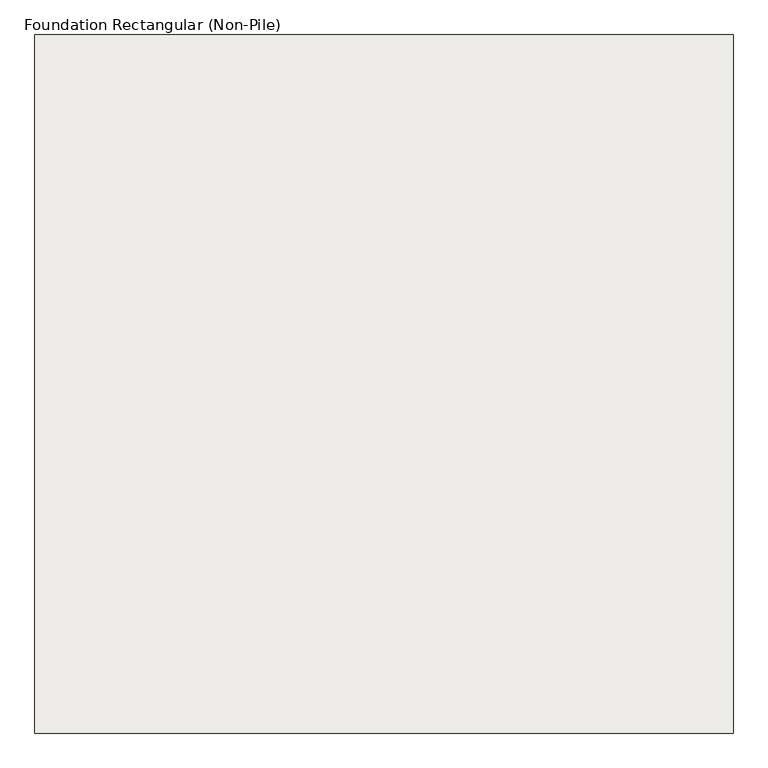
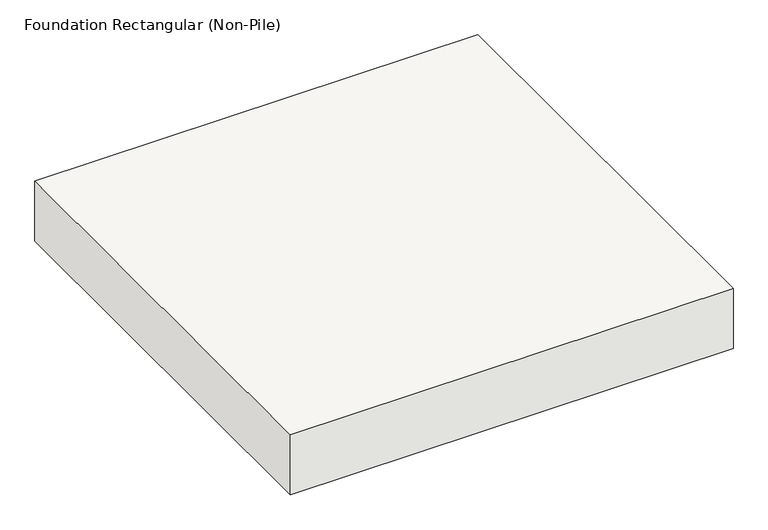
"""IFC4 building model written with IfcOpenShell, lengths in millimetres: slab geometry, Foundation Rectangular (Non-Pile) : H_SF_AR S18_Ret Fdn_F3 3500x3500x600."""

import ifcopenshell
import ifcopenshell.guid

model = None  # the IFC model being written
_history = None  # IfcOwnerHistory: only IFC2X3 demands one
_inside = {}  # id of a spatial element -> (the spatial element, [elements in it])
_under = {}  # id of a project, library or spatial element -> (it, [spatial elements below it])
_declared = {}  # id of a project -> (the project, [libraries it declares])
_typed = {}  # id of a type object -> (the type object, [elements of that type])
_made_of = {}  # id of a material, layer set ... -> (it, [elements and type objects made of it])


def new_model(schema):
    """Start an empty IFC model of exactly this schema.

    Asked for "IFC4X3", IfcOpenShell would pick the latest addendum, in which some entities
    have other attributes; the version numbers below select the first issue.
    IFC2X3 requires an IfcOwnerHistory on every rooted entity: one is made here for all.
    """
    global model, _history
    if schema == "IFC4X3":
        model = ifcopenshell.file(schema_version=(4, 3, 0, 0))
    else:
        model = ifcopenshell.file(schema=schema)
    _inside.clear()
    _under.clear()
    _declared.clear()
    _typed.clear()
    _made_of.clear()
    _history = None
    if model.schema == "IFC2X3":
        org = make("IfcOrganization", Name="unknown")
        user = make(
            "IfcPersonAndOrganization",
            ThePerson=make("IfcPerson", FamilyName="unknown"),
            TheOrganization=org,
        )
        app = make(
            "IfcApplication",
            ApplicationDeveloper=org,
            Version="unknown",
            ApplicationFullName="unknown",
            ApplicationIdentifier="unknown",
        )
        _history = make(
            "IfcOwnerHistory",
            OwningUser=user,
            OwningApplication=app,
            ChangeAction="ADDED",
            CreationDate=0,
        )
    return model


def make(cls, **values):
    """One entity of the class cls with the attributes given. An attribute that is None is left unset."""
    return model.create_entity(
        cls, **{name: value for name, value in values.items() if value is not None}
    )


def rooted(cls, **values):
    """An entity with a GlobalId (a new one), such as an element, a storey or a relation."""
    return make(cls, GlobalId=ifcopenshell.guid.new(), OwnerHistory=_history, **values)


def si_unit(unit_type, name, prefix=None):
    """IfcSIUnit, for example si_unit("LENGTHUNIT", "METRE", prefix="MILLI")."""
    return make("IfcSIUnit", UnitType=unit_type, Prefix=prefix, Name=name)


def assignment(units):
    """IfcUnitAssignment: the units of a project."""
    return None if units is None else make("IfcUnitAssignment", Units=units)


def point(xyz):
    """IfcCartesianPoint."""
    return None if xyz is None else make("IfcCartesianPoint", Coordinates=xyz)


def direction(xyz):
    """IfcDirection."""
    return None if xyz is None else make("IfcDirection", DirectionRatios=xyz)


def frame(location, z_axis=None, x_axis=None):
    """IfcAxis2Placement3D, a coordinate frame: its origin and axes. An axis left out is left unset."""
    return make(
        "IfcAxis2Placement3D",
        Location=point(location),
        Axis=direction(z_axis),
        RefDirection=direction(x_axis),
    )


def origin():
    """The frame at (0, 0, 0) with its axes left unset."""
    return frame((0.0, 0.0, 0.0))


def place(relative_to, where):
    """IfcLocalPlacement: puts the frame where relative to a parent placement (None: the world)."""
    return make(
        "IfcLocalPlacement", PlacementRelTo=relative_to, RelativePlacement=where
    )


def context(
    kind, dimensions, precision=None, world=None, true_north=None, identifier=None
):
    """IfcGeometricRepresentationContext, for example the 3D "Model" context."""
    return make(
        "IfcGeometricRepresentationContext",
        ContextIdentifier=identifier,
        ContextType=kind,
        CoordinateSpaceDimension=dimensions,
        Precision=precision,
        WorldCoordinateSystem=world,
        TrueNorth=true_north,
    )


def project(units=None, contexts=None):
    """IfcProject with its units and contexts."""
    return rooted(
        "IfcProject",
        Name="project",
        RepresentationContexts=contexts,
        UnitsInContext=assignment(units),
    )


def spatial(cls, under=None, at=None, **own):
    """A site, building, storey or space (cls), placed at a placement, below another one or the project."""
    s = rooted(cls, ObjectPlacement=at, **own)
    if under is not None:
        _under.setdefault(under.id(), (under, []))[1].append(s)
    return s


def polyline(points):
    """IfcPolyline through the points."""
    return make("IfcPolyline", Points=[point(p) for p in points])


def outline(outer, holes=None, kind="AREA"):
    """IfcArbitraryClosedProfileDef: a profile drawn as a closed curve; with holes, ...WithVoids."""
    if holes is None:
        return make("IfcArbitraryClosedProfileDef", ProfileType=kind, OuterCurve=outer)
    return make(
        "IfcArbitraryProfileDefWithVoids",
        ProfileType=kind,
        OuterCurve=outer,
        InnerCurves=holes,
    )


def extrude(swept, where, along, depth):
    """IfcExtrudedAreaSolid: the profile swept, set in the frame where, extruded along a direction by depth."""
    return make(
        "IfcExtrudedAreaSolid",
        SweptArea=swept,
        Position=where,
        ExtrudedDirection=direction(along),
        Depth=depth,
    )


def shape(context_of_items, identifier, shape_type, items):
    """IfcShapeRepresentation: the items that make up one representation, for example the "Body"."""
    return make(
        "IfcShapeRepresentation",
        ContextOfItems=context_of_items,
        RepresentationIdentifier=identifier,
        RepresentationType=shape_type,
        Items=items,
    )


def source(mapping_origin, context_of_items, identifier, shape_type, items):
    """IfcRepresentationMap: a shape defined once, which mapped items show again and again."""
    return make(
        "IfcRepresentationMap",
        MappingOrigin=mapping_origin,
        MappedRepresentation=shape(context_of_items, identifier, shape_type, items),
    )


def transform(
    local_origin,
    x_axis=None,
    y_axis=None,
    z_axis=None,
    scale=None,
    scale2=None,
    scale3=None,
    uniform=True,
):
    """IfcCartesianTransformationOperator3D, or its non-uniform kind. x_axis, y_axis, z_axis: its Axis1, 2, 3."""
    if uniform:
        return make(
            "IfcCartesianTransformationOperator3D",
            Axis1=direction(x_axis),
            Axis2=direction(y_axis),
            LocalOrigin=point(local_origin),
            Scale=scale,
            Axis3=direction(z_axis),
        )
    return make(
        "IfcCartesianTransformationOperator3DnonUniform",
        Axis1=direction(x_axis),
        Axis2=direction(y_axis),
        LocalOrigin=point(local_origin),
        Scale=scale,
        Axis3=direction(z_axis),
        Scale2=scale2,
        Scale3=scale3,
    )


def mapped(mapping_source, mapping_target):
    """IfcMappedItem: shows the shape of a source again, moved by a transform."""
    return make(
        "IfcMappedItem", MappingSource=mapping_source, MappingTarget=mapping_target
    )


def made_of(thing, what):
    """Note that an element or type object is made of a material, layer set ...; save() writes the relation."""
    if what is not None:
        _made_of.setdefault(what.id(), (what, []))[1].append(thing)
    return thing


def element(
    cls,
    number,
    at=None,
    inside=None,
    cuts=None,
    type_object=None,
    material=None,
    context=None,
    identifier="Body",
    shape_type=None,
    held_by="IfcProductDefinitionShape",
    body=None,
    shapes=None,
    **own,
):
    """One element of the class cls, such as IfcWall. Its Tag is "e" and its number.

    at: its placement. inside: the storey or other place that contains it. cuts: it is an
    opening in that element (IfcRelVoidsElement). A single representation is given by context,
    identifier, shape_type and body (its items); several are given by shapes. held_by: the class
    of the entity that holds the representations. save() writes the other relations.
    """
    e = rooted(cls, Tag="e%d" % number, ObjectPlacement=at, **own)
    if body is not None:
        shapes = [shape(context, identifier, shape_type, body)]
    if shapes is not None:
        e.Representation = make(held_by, Representations=shapes)
    if inside is not None:
        _inside.setdefault(inside.id(), (inside, []))[1].append(e)
    if cuts is not None:
        rooted(
            "IfcRelVoidsElement", RelatingBuildingElement=cuts, RelatedOpeningElement=e
        )
    if type_object is not None:
        _typed.setdefault(type_object.id(), (type_object, []))[1].append(e)
    return made_of(e, material)


def aggregate(whole, parts):
    """IfcRelAggregates: a whole, such as a stair, and the parts it consists of."""
    return rooted("IfcRelAggregates", RelatingObject=whole, RelatedObjects=parts)


def save(model, path):
    """Write the relations noted so far, then the file.

    IfcRelAggregates (storeys below a building ...), IfcRelContainedInSpatialStructure (elements
    in a storey), IfcRelDefinesByType, IfcRelAssociatesMaterial and IfcRelDeclares: one each for
    every whole, place, type object, material and project.
    """
    for whole, parts in _under.values():
        aggregate(whole, parts)
    for where, things in _inside.values():
        rooted(
            "IfcRelContainedInSpatialStructure",
            RelatedElements=things,
            RelatingStructure=where,
        )
    for kind, things in _typed.values():
        rooted("IfcRelDefinesByType", RelatedObjects=things, RelatingType=kind)
    for what, things in _made_of.values():
        rooted("IfcRelAssociatesMaterial", RelatedObjects=things, RelatingMaterial=what)
    for by, libraries in _declared.values():
        rooted("IfcRelDeclares", RelatingContext=by, RelatedDefinitions=libraries)
    model.write(path)


def foundation_rectangular_non_pile_20b31725(model_context):
    return source(origin(), model_context, "Body", "SweptSolid", [
        extrude(outline(polyline([(1750.0, 1750.0), (1750.0, -1750.0), (-1750.0, -1750.0), (-1750.0, 1750.0), (1750.0, 1750.0)])), frame((0.0, 0.0, -500.0), z_axis=(0.0, 0.0, 1.0), x_axis=(1.0, 0.0, 0.0)), (0.0, 0.0, 1.0), 500.0),
    ])


if __name__ == "__main__":
    model = new_model("IFC4")
    model_context = context("Model", 3, world=origin())
    ifc_project = project(units=[si_unit("LENGTHUNIT", "METRE", prefix="MILLI")], contexts=[model_context])
    site = spatial("IfcSite", under=ifc_project)
    building = spatial("IfcBuilding", under=site)
    placement = place(None, origin())
    foundation_rectangular_non_pile_shape = foundation_rectangular_non_pile_20b31725(model_context)
    element("IfcSlab", 1, ObjectType="Foundation Rectangular (Non-Pile) : H_SF_AR S18_Ret Fdn_F3 3500x3500x600", at=placement, inside=building, context=model_context, shape_type="MappedRepresentation", body=[
        mapped(foundation_rectangular_non_pile_shape, transform((0.0, 0.0, 0.0), x_axis=(1.0, 0.0, 0.0), y_axis=(0.0, 1.0, 0.0), z_axis=(0.0, 0.0, 1.0))),
    ])
    save(model, "model.ifc")

# Revit data of these elements
# Type "Foundation Rectangular (Non-Pile) : H_SF_AR S18_Ret Fdn_F3 3500x3500x600"
#   Type Comments = "UG"
#   Type Mark = "F3"
#   Top bar = "D25@300"
#   Description = "UG Shallow Foundation"
#   Bottom bar = "D20@300"
#   H_Rebar Ratio = 0.12
#   Width = 3500 mm
#   Length = 3500 mm
#   Foundation Thickness = 500 mm
#   Structural Material [instance default] = none
#   Assembly Code = ""
# Element 1 (IfcSlab, "Foundation Rectangular (Non-Pile) : H_SF_AR S18_Ret Fdn_F3 3500x3500x600")
#   Materials on its faces: "00_Concrete_Reinf. Conc."
# Materials
#   "00_Concrete_Reinf. Conc.": class "Concrete", colour RGB 176 176 176, transparency 0, Description = "Reinf. Conc.", Cost = 0, Image = Concrete.Cast-In-Place.Flat.Polished.Grey.jpg
